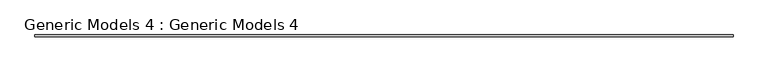
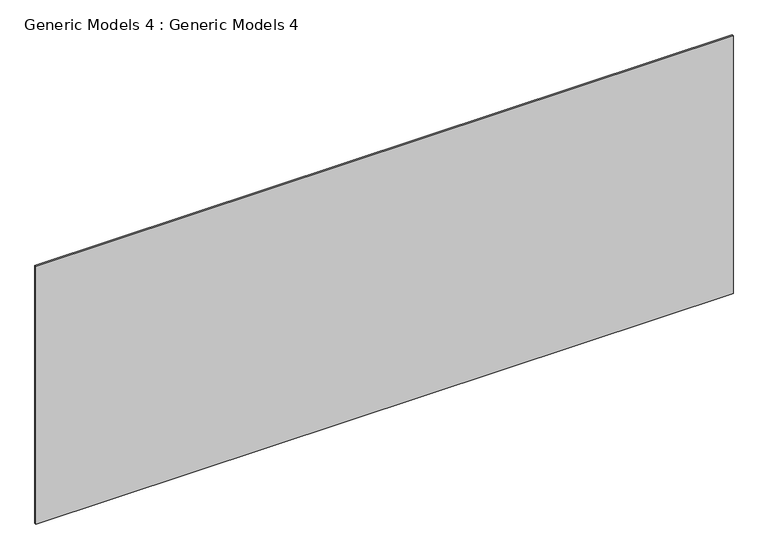
"""IFC4 building model written with IfcOpenShell, lengths in millimetres: proxy geometry, Generic Models 4 : Generic Models 4."""

from ifc_helpers import new_model, si_unit, frame, origin, place, context, project, spatial, polyline, outline, extrude, source, transform, mapped, element, save


def generic_models_4_generic_models_4_eadb5206(model_context):
    return source(origin(), model_context, "Body", "SweptSolid", [
        extrude(outline(polyline([(0.0, -15.875), (0.0, 0.0), (6189.931498, 0.0), (6189.931498, -15.875), (0.0, -15.875)])), frame((8386.8578684, -6915.7230338, 124059.696), z_axis=(0.0, -1.0913936421275393e-12, 1.0), x_axis=(-1.0, 0.0, 0.0)), (0.0, 0.0, 1.0), 2419.35),
    ])


if __name__ == "__main__":
    model = new_model("IFC4")
    model_context = context("Model", 3, world=origin())
    ifc_project = project(units=[si_unit("LENGTHUNIT", "METRE", prefix="MILLI")], contexts=[model_context])
    site = spatial("IfcSite", under=ifc_project)
    building = spatial("IfcBuilding", under=site)
    placement = place(None, origin())
    generic_models_4_generic_models_4_shape = generic_models_4_generic_models_4_eadb5206(model_context)
    element("IfcBuildingElementProxy", 1, Name="Generic Models 4 : Generic Models 4", ObjectType="Generic Models 4 : Generic Models 4", at=placement, inside=building, context=model_context, shape_type="MappedRepresentation", body=[
        mapped(generic_models_4_generic_models_4_shape, transform((0.0, 0.0, 0.0), x_axis=(1.0, 0.0, 0.0), y_axis=(0.0, 1.0, 0.0), z_axis=(0.0, 0.0, 1.0))),
    ])
    save(model, "model.ifc")

# Revit data of these elements
# Element 1 (IfcBuildingElementProxy, "Generic Models 4 : Generic Models 4")
#   Materials on its faces: "_5/8\" DRYWALL"
# Materials
#   "_5/8\" DRYWALL": class "Generic", colour RGB 191 191 191, transparency 0, Cost = 0
